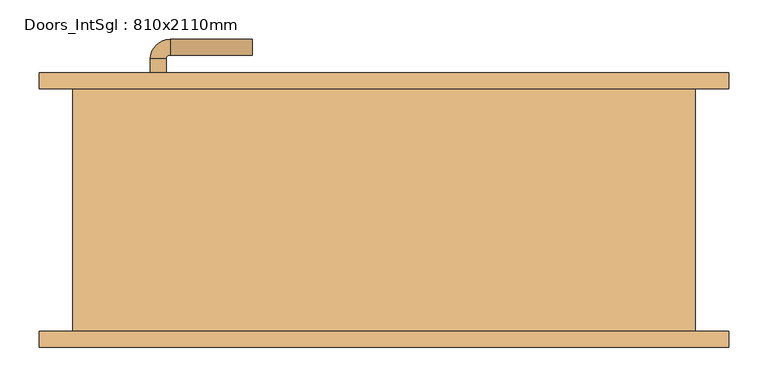
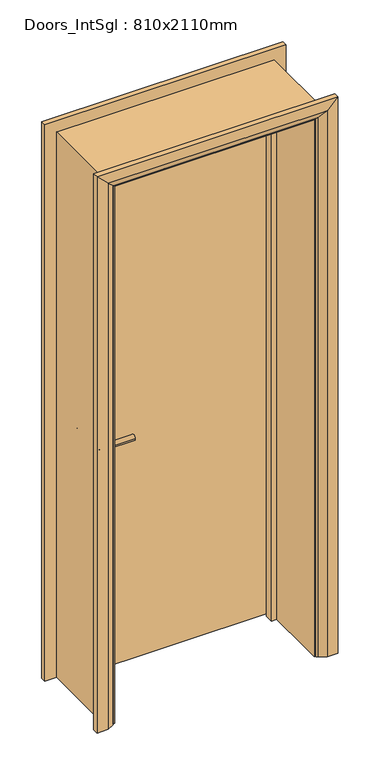
"""IFC4 building model written with IfcOpenShell, lengths in millimetres: door geometry, Doors_IntSgl : 810x2110mm."""

from ifc_helpers import new_model, si_unit, point, frame, frame_2d, origin, place, context, project, spatial, polyline, circle_curve, ellipse_curve, trimmed, segment, composite_curve, outline, extrude, faceted_brep, source, transform, mapped, element, save
from ifc_brep_helpers import plane_surface, cylinder_surface, revolved_surface, advanced_brep


def doors_intsgl_810x2110mm_01ce896d(model_context):
    return source(origin(), model_context, "Body", "SolidModel", [
        advanced_brep(
        [(-298.0, 109.0, 900.0), (-278.0, 109.0, 900.0), (-278.0, 79.0, 900.0), (-298.0, 79.0, 900.0), (-273.0, 74.0, 900.0), (-273.0, 54.0, 900.0), (-168.0, 54.0, 900.0), (-168.0, 74.0, 900.0)],
        [
            (0, 1, circle_curve(frame((-288.0, 109.0, 900.0), z_axis=(0.0, 1.0, 0.0), x_axis=(1.0, 0.0, 0.0)), 10.0)),
            (1, 0, circle_curve(frame((-288.0, 109.0, 900.0), z_axis=(0.0, 1.0, 0.0), x_axis=(1.0, 0.0, 0.0)), 10.0)),
            (1, 2),
            (2, 3, circle_curve(frame((-288.0, 79.0, 900.0), z_axis=(0.0, 1.0, 0.0), x_axis=(1.0, 0.0, 0.0)), 10.0)),
            (3, 0),
            (3, 2, circle_curve(frame((-288.0, 79.0, 900.0), z_axis=(0.0, 1.0, 0.0), x_axis=(1.0, 0.0, 0.0)), 10.0)),
            (4, 5, circle_curve(frame((-273.0, 64.0, 900.0), z_axis=(-1.0, 0.0, 0.0), x_axis=(0.0, 1.0, 0.0)), 10.0)),
            (5, 3, circle_curve(frame((-273.0, 79.0, 900.0), z_axis=(0.0, 0.0, -1.0), x_axis=(-1.0, 0.0, 0.0)), 25.0)),
            (2, 4, circle_curve(frame((-273.0, 79.0, 900.0), z_axis=(0.0, 0.0, 1.0), x_axis=(-1.0, 0.0, 0.0)), 5.0)),
            (5, 4, circle_curve(frame((-273.0, 64.0, 900.0), z_axis=(-1.0, 0.0, 0.0), x_axis=(0.0, 1.0, 0.0)), 10.0)),
            (6, 7, circle_curve(frame((-168.0, 64.0, 900.0), z_axis=(1.0, 0.0, 0.0), x_axis=(0.0, 1.0, 0.0)), 10.0)),
            (7, 6, circle_curve(frame((-168.0, 64.0, 900.0), z_axis=(1.0, 0.0, 0.0), x_axis=(0.0, 1.0, 0.0)), 10.0)),
            (4, 7),
            (6, 5),
        ],
        [
            plane_surface(frame((-288.0, 109.0, 900.0), z_axis=(0.0, 1.0, 0.0), x_axis=(0.0, 0.0, 1.0))),
            cylinder_surface(frame((-288.0, 109.0, 900.0), z_axis=(0.0, 1.0, 0.0), x_axis=(1.0, 0.0, 0.0)), 10.0),
            revolved_surface(trimmed(ellipse_curve(frame((-288.0, 79.0, 900.0), z_axis=(0.0, -1.0, 0.0), x_axis=(1.0, 0.0, 0.0)), 10.0, 10.0), [point((-298.0, 79.0, 900.0))], [point((-278.0, 79.0, 900.0))], True, "CARTESIAN"), (-273.0, 79.0, 900.0), (0.0, 0.0, -1.0)),
            revolved_surface(trimmed(ellipse_curve(frame((-288.0, 79.0, 900.0), z_axis=(0.0, -1.0, 0.0), x_axis=(1.0, 0.0, 0.0)), 10.0, 10.0), [point((-278.0, 79.0, 900.0))], [point((-298.0, 79.0, 900.0))], True, "CARTESIAN"), (-273.0, 79.0, 900.0), (0.0, 0.0, -1.0)),
            plane_surface(frame((-168.0, 64.0, 900.0), z_axis=(1.0, 0.0, 0.0), x_axis=(0.0, 0.0, 1.0))),
            cylinder_surface(frame((-273.0, 64.0, 900.0), z_axis=(-1.0, 0.0, 0.0), x_axis=(0.0, 1.0, 0.0)), 10.0),
        ],
        [
            (0, [[1, 2]]),
            (1, [[3, 4, 5, -2]]),
            (1, [[-5, 6, -3, -1]]),
            (2, [[7, 8, -4, 9]]),
            (3, [[10, -9, -6, -8]]),
            (4, [[11, 12]]),
            (5, [[13, -11, 14, -7]]),
            (5, [[-14, -12, -13, -10]]),
        ],
    ),
        extrude(outline(composite_curve([segment(trimmed(circle_curve(frame_2d((900.0, -290.5)), 30.0), [point((900.0, -320.5))], [point((900.0, -260.5))], False, "CARTESIAN"), True, "CONTINUOUS"), segment(trimmed(circle_curve(frame_2d((900.0, -290.5)), 30.0), [point((900.0, -260.5))], [point((900.0, -320.5))], False, "CARTESIAN"), True, "CONTINUOUS")], self_intersect=False)), frame((0.0, 109.0, 0.0), z_axis=(0.0, 1.0, 0.0), x_axis=(0.0, 0.0, 1.0)), (0.0, 0.0, 1.0), 8.0),
        advanced_brep(
        [(-298.0, 163.0, 900.0), (-278.0, 163.0, 900.0), (-298.0, 193.0, 900.0), (-278.0, 193.0, 900.0), (-273.0, 198.0, 900.0), (-273.0, 218.0, 900.0), (-168.0, 218.0, 900.0), (-168.0, 198.0, 900.0)],
        [
            (0, 1, circle_curve(frame((-288.0, 163.0, 900.0), z_axis=(0.0, -1.0, 0.0), x_axis=(1.0, 0.0, 0.0)), 10.0)),
            (1, 0, circle_curve(frame((-288.0, 163.0, 900.0), z_axis=(0.0, -1.0, 0.0), x_axis=(1.0, 0.0, 0.0)), 10.0)),
            (0, 2),
            (2, 3, circle_curve(frame((-288.0, 193.0, 900.0), z_axis=(0.0, -1.0, 0.0), x_axis=(1.0, 0.0, 0.0)), 10.0)),
            (3, 1),
            (3, 2, circle_curve(frame((-288.0, 193.0, 900.0), z_axis=(0.0, -1.0, 0.0), x_axis=(1.0, 0.0, 0.0)), 10.0)),
            (4, 3, circle_curve(frame((-273.0, 193.0, 900.0), z_axis=(0.0, 0.0, 1.0), x_axis=(-1.0, 0.0, 0.0)), 5.0)),
            (2, 5, circle_curve(frame((-273.0, 193.0, 900.0), z_axis=(0.0, 0.0, -1.0), x_axis=(-1.0, 0.0, 0.0)), 25.0)),
            (5, 4, circle_curve(frame((-273.0, 208.0, 900.0), z_axis=(-1.0, 0.0, 0.0), x_axis=(0.0, -1.0, 0.0)), 10.0)),
            (4, 5, circle_curve(frame((-273.0, 208.0, 900.0), z_axis=(-1.0, 0.0, 0.0), x_axis=(0.0, -1.0, 0.0)), 10.0)),
            (6, 7, circle_curve(frame((-168.0, 208.0, 900.0), z_axis=(1.0, 0.0, 0.0), x_axis=(0.0, -1.0, 0.0)), 10.0)),
            (7, 6, circle_curve(frame((-168.0, 208.0, 900.0), z_axis=(1.0, 0.0, 0.0), x_axis=(0.0, -1.0, 0.0)), 10.0)),
            (5, 6),
            (7, 4),
        ],
        [
            plane_surface(frame((-288.0, 163.0, 900.0), z_axis=(0.0, -1.0, 0.0), x_axis=(0.0, 0.0, 1.0))),
            cylinder_surface(frame((-288.0, 163.0, 900.0), z_axis=(0.0, -1.0, 0.0), x_axis=(1.0, 0.0, 0.0)), 10.0),
            revolved_surface(trimmed(ellipse_curve(frame((-288.0, 193.0, 900.0), z_axis=(0.0, -1.0, 0.0), x_axis=(1.0, 0.0, 0.0)), 10.0, 10.0), [point((-298.0, 193.0, 900.0))], [point((-278.0, 193.0, 900.0))], True, "CARTESIAN"), (-273.0, 193.0, 900.0), (0.0, 0.0, -1.0)),
            revolved_surface(trimmed(ellipse_curve(frame((-288.0, 193.0, 900.0), z_axis=(0.0, -1.0, 0.0), x_axis=(1.0, 0.0, 0.0)), 10.0, 10.0), [point((-278.0, 193.0, 900.0))], [point((-298.0, 193.0, 900.0))], True, "CARTESIAN"), (-273.0, 193.0, 900.0), (0.0, 0.0, -1.0)),
            plane_surface(frame((-168.0, 208.0, 900.0), z_axis=(1.0, 0.0, 0.0), x_axis=(0.0, 0.0, 1.0))),
            cylinder_surface(frame((-273.0, 208.0, 900.0), z_axis=(-1.0, 0.0, 0.0), x_axis=(0.0, -1.0, 0.0)), 10.0),
        ],
        [
            (0, [[1, 2]]),
            (1, [[-1, 3, 4, 5]]),
            (1, [[-2, -5, 6, -3]]),
            (2, [[7, -4, 8, 9]]),
            (3, [[-8, -6, -7, 10]]),
            (4, [[11, 12]]),
            (5, [[-9, 13, -12, 14]]),
            (5, [[-10, -14, -11, -13]]),
        ],
    ),
        extrude(outline(composite_curve([segment(trimmed(circle_curve(frame_2d((900.0, -290.5)), 30.0), [point((900.0, -320.5))], [point((900.0, -260.5))], False, "CARTESIAN"), True, "CONTINUOUS"), segment(trimmed(circle_curve(frame_2d((900.0, -290.5)), 30.0), [point((900.0, -260.5))], [point((900.0, -320.5))], False, "CARTESIAN"), True, "CONTINUOUS")], self_intersect=False)), frame((0.0, 155.0, 0.0), z_axis=(0.0, 1.0, 0.0), x_axis=(0.0, 0.0, 1.0)), (0.0, 0.0, 1.0), 8.0),
        extrude(outline(polyline([(363.0, 117.0), (-363.0, 117.0), (-363.0, 155.0), (363.0, 155.0), (363.0, 117.0)])), frame((0.0, 0.0, 8.0), z_axis=(0.0, 0.0, 1.0), x_axis=(1.0, 0.0, 0.0)), (0.0, 0.0, 1.0), 2060.0),
        advanced_brep(
        [(440.0, 175.0, 0.0), (440.0, 155.0, 0.0), (370.0, 155.0, 0.0), (374.0, 161.0, 0.0), (400.0, 175.0, 0.0), (440.0, 175.0, 2145.0), (440.0, 155.0, 2145.0), (-440.0, 155.0, 2145.0), (-440.0, 155.0, 0.0), (-370.0, 155.0, 0.0), (-370.0, 155.0, 2075.0), (370.0, 155.0, 2075.0), (374.0, 161.0, 2079.0), (400.0, 175.0, 2105.0), (-400.0, 175.0, 2105.0), (-400.0, 175.0, 0.0), (-440.0, 175.0, 0.0), (-440.0, 175.0, 2145.0), (-374.0, 161.0, 2079.0), (-374.0, 161.0, 0.0)],
        [
            (0, 1),
            (1, 2),
            (2, 3, circle_curve(frame((378.0, 154.0, 0.0), z_axis=(0.0, 0.0, -1.0), x_axis=(1.0, 0.0, 0.0)), 8.0622577)),
            (3, 4),
            (4, 0),
            (0, 5),
            (5, 6),
            (6, 1),
            (6, 7),
            (7, 8),
            (8, 9),
            (9, 10),
            (10, 11),
            (11, 2),
            (11, 12, ellipse_curve(frame((378.0, 154.0, 2083.0), z_axis=(0.7071067811865475, 0.0, -0.7071067811865475), x_axis=(-0.7071067811865474, 0.0, -0.7071067811865476)), 11.4017543, 8.0622577)),
            (12, 3),
            (12, 13),
            (13, 4),
            (13, 14),
            (14, 15),
            (15, 16),
            (16, 17),
            (17, 5),
            (17, 7),
            (10, 18, ellipse_curve(frame((-378.0, 154.0, 2083.0), z_axis=(0.7071067811865475, 0.0, 0.7071067811865475), x_axis=(0.7071067811865476, 0.0, -0.7071067811865474)), 11.4017543, 8.0622577)),
            (18, 12),
            (18, 14),
            (15, 19),
            (19, 9, circle_curve(frame((-378.0, 154.0, 0.0), z_axis=(0.0, 0.0, -1.0), x_axis=(-1.0, 0.0, 0.0)), 8.0622577)),
            (8, 16),
            (19, 18),
        ],
        [
            plane_surface(frame((370.0, 155.0, 0.0), z_axis=(0.0, 0.0, -1.0), x_axis=(0.0, -1.0, 0.0))),
            plane_surface(frame((440.0, 175.0, 0.0), z_axis=(1.0, 0.0, 0.0), x_axis=(0.0, 0.0, 1.0))),
            plane_surface(frame((440.0, 155.0, 0.0), z_axis=(0.0, -1.0, 0.0), x_axis=(0.0, 0.0, 1.0))),
            cylinder_surface(frame((378.0, 154.0, 0.0), z_axis=(0.0, 0.0, -1.0), x_axis=(1.0, 0.0, 0.0)), 8.0622577),
            plane_surface(frame((374.0, 161.0, 0.0), z_axis=(-0.4740998230350126, 0.880471099922178, 0.0), x_axis=(0.0, 0.0, 1.0))),
            plane_surface(frame((400.0, 175.0, 0.0), z_axis=(0.0, 1.0, 0.0), x_axis=(0.0, 0.0, 1.0))),
            plane_surface(frame((440.0, 175.0, 2145.0), z_axis=(0.0, 0.0, 1.0), x_axis=(-1.0, 0.0, 0.0))),
            cylinder_surface(frame((370.0, 154.0, 2083.0), z_axis=(1.0, 0.0, 0.0), x_axis=(0.0, 0.0, 1.0)), 8.0622577),
            plane_surface(frame((374.0, 161.0, 2079.0), z_axis=(0.0, 0.8804710999221764, -0.4740998230350154), x_axis=(-1.0, 0.0, 0.0))),
            plane_surface(frame((-370.0, 155.0, 0.0), z_axis=(0.0, 0.0, -1.0), x_axis=(0.0, -1.0, 0.0))),
            plane_surface(frame((-440.0, 175.0, 2145.0), z_axis=(-1.0, 0.0, 0.0), x_axis=(0.0, 0.0, -1.0))),
            cylinder_surface(frame((-378.0, 154.0, 2075.0), z_axis=(0.0, 0.0, 1.0), x_axis=(-1.0, 0.0, 0.0)), 8.0622577),
            plane_surface(frame((-374.0, 161.0, 2079.0), z_axis=(0.47409982303501824, 0.8804710999221749, 0.0), x_axis=(0.0, 0.0, -1.0))),
        ],
        [
            (0, [[1, 2, 3, 4, 5]]),
            (1, [[-1, 6, 7, 8]]),
            (2, [[-2, -8, 9, 10, 11, 12, 13, 14]]),
            (3, [[-3, -14, 15, 16]]),
            (4, [[-4, -16, 17, 18]]),
            (5, [[-5, -18, 19, 20, 21, 22, 23, -6]]),
            (6, [[-7, -23, 24, -9]]),
            (7, [[-15, -13, 25, 26]]),
            (8, [[-17, -26, 27, -19]]),
            (9, [[-21, 28, 29, -11, 30]]),
            (10, [[-24, -22, -30, -10]]),
            (11, [[-25, -12, -29, 31]]),
            (12, [[-27, -31, -28, -20]]),
        ],
    ),
        extrude(outline(polyline([(0.0, -365.0), (0.0, -346.0), (2051.0, -346.0), (2051.0, 346.0), (0.0, 346.0), (0.0, 365.0), (2070.0, 365.0), (2070.0, -365.0), (0.0, -365.0)])), frame((0.0, 83.0, 0.0), z_axis=(0.0, 1.0, 0.0), x_axis=(0.0, 0.0, 1.0)), (0.0, 0.0, 1.0), 32.0),
        advanced_brep(
        [(-440.0, -175.0, 0.0), (-440.0, -155.0, 0.0), (-370.0, -155.0, 0.0), (-374.0, -161.0, 0.0), (-400.0, -175.0, 0.0), (-440.0, -175.0, 2145.0), (-440.0, -155.0, 2145.0), (-370.0, -155.0, 2075.0), (-374.0, -161.0, 2079.0), (-400.0, -175.0, 2105.0), (440.0, -175.0, 2145.0), (440.0, -155.0, 2145.0), (370.0, -155.0, 2075.0), (374.0, -161.0, 2079.0), (400.0, -175.0, 2105.0), (440.0, -175.0, 0.0), (400.0, -175.0, 0.0), (374.0, -161.0, 0.0), (370.0, -155.0, 0.0), (440.0, -155.0, 0.0)],
        [
            (0, 1),
            (1, 2),
            (2, 3, circle_curve(frame((-378.0, -154.0, 0.0), z_axis=(0.0, 0.0, -1.0), x_axis=(-1.0, 0.0, 0.0)), 8.0622577)),
            (3, 4),
            (4, 0),
            (0, 5),
            (5, 6),
            (6, 1),
            (6, 7),
            (7, 2),
            (7, 8, ellipse_curve(frame((-378.0, -154.0, 2083.0), z_axis=(-0.7071067811865475, 0.0, -0.7071067811865475), x_axis=(0.7071067811865474, 0.0, -0.7071067811865476)), 11.4017543, 8.0622577)),
            (8, 3),
            (8, 9),
            (9, 4),
            (9, 5),
            (5, 10),
            (10, 11),
            (11, 6),
            (11, 12),
            (12, 7),
            (12, 13, ellipse_curve(frame((378.0, -154.0, 2083.0), z_axis=(-0.7071067811865475, 0.0, 0.7071067811865475), x_axis=(-0.7071067811865476, 0.0, -0.7071067811865474)), 11.4017543, 8.0622577)),
            (13, 8),
            (13, 14),
            (14, 9),
            (14, 10),
            (15, 16),
            (16, 17),
            (17, 18, circle_curve(frame((378.0, -154.0, 0.0), z_axis=(0.0, 0.0, -1.0), x_axis=(1.0, 0.0, 0.0)), 8.0622577)),
            (18, 19),
            (19, 15),
            (10, 15),
            (19, 11),
            (18, 12),
            (17, 13),
            (16, 14),
        ],
        [
            plane_surface(frame((-370.0, -227.8010989, 0.0), z_axis=(0.0, 0.0, -1.0), x_axis=(1.0, 0.0, 0.0))),
            plane_surface(frame((-440.0, -175.0, 0.0), z_axis=(-1.0, 0.0, 0.0), x_axis=(0.0, 0.0, 1.0))),
            plane_surface(frame((-440.0, -155.0, 0.0), z_axis=(0.0, 1.0, 0.0), x_axis=(0.0, 0.0, 1.0))),
            cylinder_surface(frame((-378.0, -154.0, 0.0), z_axis=(0.0, 0.0, -1.0), x_axis=(-1.0, 0.0, 0.0)), 8.0622577),
            plane_surface(frame((-374.0, -161.0, 0.0), z_axis=(0.4740998230350183, -0.8804710999221749, 0.0), x_axis=(0.0, 0.0, 1.0))),
            plane_surface(frame((-400.0, -175.0, 0.0), z_axis=(0.0, -1.0, 0.0), x_axis=(0.0, 0.0, 1.0))),
            plane_surface(frame((-440.0, -175.0, 2145.0), z_axis=(0.0, 0.0, 1.0), x_axis=(1.0, 0.0, 0.0))),
            plane_surface(frame((-440.0, -155.0, 2145.0), z_axis=(0.0, 1.0, 0.0), x_axis=(1.0, 0.0, 0.0))),
            cylinder_surface(frame((-370.0, -154.0, 2083.0), z_axis=(-1.0, 0.0, 0.0), x_axis=(0.0, 0.0, 1.0)), 8.0622577),
            plane_surface(frame((-374.0, -161.0, 2079.0), z_axis=(0.0, -0.8804710999221749, -0.4740998230350183), x_axis=(1.0, 0.0, 0.0))),
            plane_surface(frame((-400.0, -175.0, 2105.0), z_axis=(0.0, -1.0, 0.0), x_axis=(1.0, 0.0, 0.0))),
            plane_surface(frame((370.0, -227.8010989, 0.0), z_axis=(0.0, 0.0, -1.0), x_axis=(-1.0, 0.0, 0.0))),
            plane_surface(frame((440.0, -175.0, 2145.0), z_axis=(1.0, 0.0, 0.0), x_axis=(0.0, 0.0, -1.0))),
            plane_surface(frame((440.0, -155.0, 2145.0), z_axis=(0.0, 1.0, 0.0), x_axis=(0.0, 0.0, -1.0))),
            cylinder_surface(frame((378.0, -154.0, 2075.0), z_axis=(0.0, 0.0, 1.0), x_axis=(1.0, 0.0, 0.0)), 8.0622577),
            plane_surface(frame((374.0, -161.0, 2079.0), z_axis=(-0.4740998230350183, -0.8804710999221749, 0.0), x_axis=(0.0, 0.0, -1.0))),
            plane_surface(frame((400.0, -175.0, 2105.0), z_axis=(0.0, -1.0, 0.0), x_axis=(0.0, 0.0, -1.0))),
        ],
        [
            (0, [[1, 2, 3, 4, 5]]),
            (1, [[-1, 6, 7, 8]]),
            (2, [[-2, -8, 9, 10]]),
            (3, [[-3, -10, 11, 12]]),
            (4, [[-4, -12, 13, 14]]),
            (5, [[-5, -14, 15, -6]]),
            (6, [[-7, 16, 17, 18]]),
            (7, [[-9, -18, 19, 20]]),
            (8, [[-11, -20, 21, 22]]),
            (9, [[-13, -22, 23, 24]]),
            (10, [[-15, -24, 25, -16]]),
            (11, [[26, 27, 28, 29, 30]]),
            (12, [[-17, 31, -30, 32]]),
            (13, [[-19, -32, -29, 33]]),
            (14, [[-21, -33, -28, 34]]),
            (15, [[-23, -34, -27, 35]]),
            (16, [[-25, -35, -26, -31]]),
        ],
    ),
        faceted_brep([(-365.0, 155.0, 0.0), (-365.0, -155.0, 0.0), (-397.0, -155.0, 0.0), (-397.0, 155.0, 0.0), (-365.0, 155.0, 2070.0), (-365.0, -155.0, 2070.0), (-397.0, -155.0, 2102.0), (-397.0, 155.0, 2102.0), (365.0, 155.0, 2070.0), (365.0, -155.0, 2070.0), (397.0, -155.0, 2102.0), (397.0, 155.0, 2102.0), (365.0, 155.0, 0.0), (397.0, 155.0, 0.0), (397.0, -155.0, 0.0), (365.0, -155.0, 0.0)], [[[0, 1, 2, 3]], [[1, 0, 4, 5]], [[2, 1, 5, 6]], [[3, 2, 6, 7]], [[0, 3, 7, 4]], [[5, 4, 8, 9]], [[6, 5, 9, 10]], [[7, 6, 10, 11]], [[4, 7, 11, 8]], [[12, 13, 14, 15]], [[9, 8, 12, 15]], [[10, 9, 15, 14]], [[11, 10, 14, 13]], [[8, 11, 13, 12]]]),
    ])


if __name__ == "__main__":
    model = new_model("IFC4")
    model_context = context("Model", 3, world=origin())
    ifc_project = project(units=[si_unit("LENGTHUNIT", "METRE", prefix="MILLI")], contexts=[model_context])
    site = spatial("IfcSite", under=ifc_project)
    building = spatial("IfcBuilding", under=site)
    placement = place(None, origin())
    doors_intsgl_810x2110mm_shape = doors_intsgl_810x2110mm_01ce896d(model_context)
    element("IfcDoor", 1, ObjectType="Doors_IntSgl : 810x2110mm", at=placement, inside=building, context=model_context, shape_type="MappedRepresentation", body=[
        mapped(doors_intsgl_810x2110mm_shape, transform((0.0, 0.0, 0.0), x_axis=(1.0, 0.0, 0.0), y_axis=(0.0, 1.0, 0.0), z_axis=(0.0, 0.0, 1.0))),
    ])
    save(model, "model.ifc")

# Revit data of these elements
# Project information
#   Workset = "Project Info"
#   Project Issue Date = "Issue Date"
#   Project Status = "Project Status"
#   Client Name = "Owner"
#   Project Address = "Enter address here"
#   Project Name = "Project Name"
#   Project Number = "Project Number"
# Type "Doors_IntSgl : 810x2110mm"
#   Construction Type Id = "MDOOR"
#   Type Mark = "42"
#   Type Comments = "Internal Single"
#   Operation = "SingleSwingRight"
#   Manufacturer = "Revit"
#   Keynote = "L20"
#   Description = "Internal Single Door"
#   Analytic Construction = "Metal"
#   UnderCut = 8 mm
#   Tolerance = 2 mm
#   Thickness = 38 mm
#   Thermal Resistance (R) = 0.270117 (m²·K)/W
#   Structural Tolerance = 8 mm
#   StopDepth = 32 mm
#   Stop Thickness = 19 mm
#   Rough Width = 810 mm
#   Rough Height = 2110 mm
#   Height to Top Lock Rail = 1000 mm
#   Heat Transfer Coefficient (U) = 3.7021 W/(m²·K)
#   Handle Z Distance = 900 mm
#   Handle X Distance = 75 mm
#   Frame Thickness = 32 mm
#   Door Panel Width = 726 mm
#   Door Panel Thickness = 38 mm
#   Door Panel Offset = 0 mm
#   Height = 2110 mm
#   Width = 810 mm
#   Door Panel Height = 2060 mm
#   Architrave Setback = 5 mm
#   Define Thermal Properties by = 1
#   Vis - Ironmongery = yes
#   Material Ironmongery = Door - Handle
#   Material Frame = Door - Frame/Mullion (1)
#   Material Door = Door - Panel
#   Material Architrave = Door - Architrave
#   Visual Light Transmittance = 0
#   Solar Heat Gain Coefficient = 0
#   Function = (empty or 0)
#   Wall Closure = (empty or 0)
# Element 1 (IfcDoor, "Doors_IntSgl : 810x2110mm")
#   Materials on its faces: "Door - Architrave", "Door - Handle", "Door - Frame/Mullion (1)", "Door - Panel"
# Materials
#   "Door - Handle": class "Miscellaneous", colour RGB 0 0 0, transparency 0, Keynote = "P21", Cost = 0
#   "Door - Frame/Mullion (1)": class "Wood", colour RGB 212 179 113, transparency 0, Keynote = "L20", Cost = 0
#   "Door - Panel": class "Wood", colour RGB 210 159 95, transparency 0, Keynote = "L20", Cost = 0
#   "Door - Architrave": class "Wood", colour RGB 154 90 5, transparency 0, Keynote = "P20", Cost = 0
